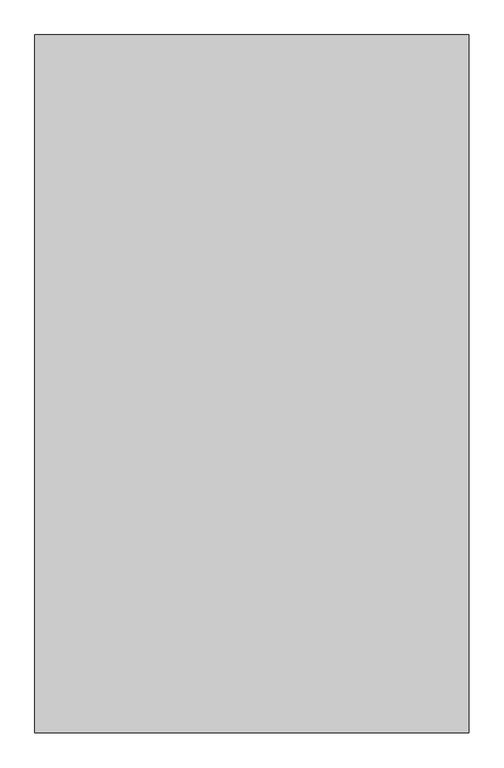
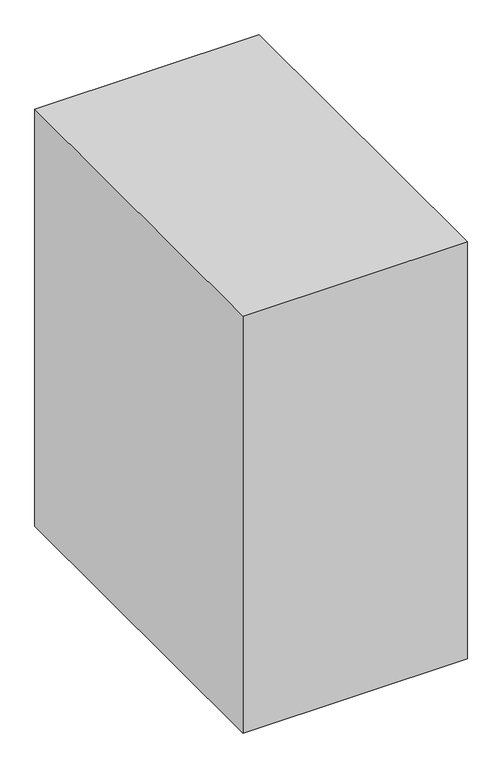
"""IFC4 building model written with IfcOpenShell, lengths in millimetres: proxy geometry, Space Planning Box_hec : Space Planning Box_hec."""

import ifcopenshell
import ifcopenshell.guid

model = None  # the IFC model being written
_history = None  # IfcOwnerHistory: only IFC2X3 demands one
_inside = {}  # id of a spatial element -> (the spatial element, [elements in it])
_under = {}  # id of a project, library or spatial element -> (it, [spatial elements below it])
_declared = {}  # id of a project -> (the project, [libraries it declares])
_typed = {}  # id of a type object -> (the type object, [elements of that type])
_made_of = {}  # id of a material, layer set ... -> (it, [elements and type objects made of it])


def new_model(schema):
    """Start an empty IFC model of exactly this schema.

    Asked for "IFC4X3", IfcOpenShell would pick the latest addendum, in which some entities
    have other attributes; the version numbers below select the first issue.
    IFC2X3 requires an IfcOwnerHistory on every rooted entity: one is made here for all.
    """
    global model, _history
    if schema == "IFC4X3":
        model = ifcopenshell.file(schema_version=(4, 3, 0, 0))
    else:
        model = ifcopenshell.file(schema=schema)
    _inside.clear()
    _under.clear()
    _declared.clear()
    _typed.clear()
    _made_of.clear()
    _history = None
    if model.schema == "IFC2X3":
        org = make("IfcOrganization", Name="unknown")
        user = make(
            "IfcPersonAndOrganization",
            ThePerson=make("IfcPerson", FamilyName="unknown"),
            TheOrganization=org,
        )
        app = make(
            "IfcApplication",
            ApplicationDeveloper=org,
            Version="unknown",
            ApplicationFullName="unknown",
            ApplicationIdentifier="unknown",
        )
        _history = make(
            "IfcOwnerHistory",
            OwningUser=user,
            OwningApplication=app,
            ChangeAction="ADDED",
            CreationDate=0,
        )
    return model


def make(cls, **values):
    """One entity of the class cls with the attributes given. An attribute that is None is left unset."""
    return model.create_entity(
        cls, **{name: value for name, value in values.items() if value is not None}
    )


def rooted(cls, **values):
    """An entity with a GlobalId (a new one), such as an element, a storey or a relation."""
    return make(cls, GlobalId=ifcopenshell.guid.new(), OwnerHistory=_history, **values)


def si_unit(unit_type, name, prefix=None):
    """IfcSIUnit, for example si_unit("LENGTHUNIT", "METRE", prefix="MILLI")."""
    return make("IfcSIUnit", UnitType=unit_type, Prefix=prefix, Name=name)


def assignment(units):
    """IfcUnitAssignment: the units of a project."""
    return None if units is None else make("IfcUnitAssignment", Units=units)


def point(xyz):
    """IfcCartesianPoint."""
    return None if xyz is None else make("IfcCartesianPoint", Coordinates=xyz)


def direction(xyz):
    """IfcDirection."""
    return None if xyz is None else make("IfcDirection", DirectionRatios=xyz)


def frame(location, z_axis=None, x_axis=None):
    """IfcAxis2Placement3D, a coordinate frame: its origin and axes. An axis left out is left unset."""
    return make(
        "IfcAxis2Placement3D",
        Location=point(location),
        Axis=direction(z_axis),
        RefDirection=direction(x_axis),
    )


def origin():
    """The frame at (0, 0, 0) with its axes left unset."""
    return frame((0.0, 0.0, 0.0))


def origin_with_axes():
    """The frame at (0, 0, 0) with the z axis (0, 0, 1) and the x axis (1, 0, 0) written out."""
    return frame((0.0, 0.0, 0.0), z_axis=(0.0, 0.0, 1.0), x_axis=(1.0, 0.0, 0.0))


def place(relative_to, where):
    """IfcLocalPlacement: puts the frame where relative to a parent placement (None: the world)."""
    return make(
        "IfcLocalPlacement", PlacementRelTo=relative_to, RelativePlacement=where
    )


def context(
    kind, dimensions, precision=None, world=None, true_north=None, identifier=None
):
    """IfcGeometricRepresentationContext, for example the 3D "Model" context."""
    return make(
        "IfcGeometricRepresentationContext",
        ContextIdentifier=identifier,
        ContextType=kind,
        CoordinateSpaceDimension=dimensions,
        Precision=precision,
        WorldCoordinateSystem=world,
        TrueNorth=true_north,
    )


def project(units=None, contexts=None):
    """IfcProject with its units and contexts."""
    return rooted(
        "IfcProject",
        Name="project",
        RepresentationContexts=contexts,
        UnitsInContext=assignment(units),
    )


def spatial(cls, under=None, at=None, **own):
    """A site, building, storey or space (cls), placed at a placement, below another one or the project."""
    s = rooted(cls, ObjectPlacement=at, **own)
    if under is not None:
        _under.setdefault(under.id(), (under, []))[1].append(s)
    return s


def polyline(points):
    """IfcPolyline through the points."""
    return make("IfcPolyline", Points=[point(p) for p in points])


def outline(outer, holes=None, kind="AREA"):
    """IfcArbitraryClosedProfileDef: a profile drawn as a closed curve; with holes, ...WithVoids."""
    if holes is None:
        return make("IfcArbitraryClosedProfileDef", ProfileType=kind, OuterCurve=outer)
    return make(
        "IfcArbitraryProfileDefWithVoids",
        ProfileType=kind,
        OuterCurve=outer,
        InnerCurves=holes,
    )


def extrude(swept, where, along, depth):
    """IfcExtrudedAreaSolid: the profile swept, set in the frame where, extruded along a direction by depth."""
    return make(
        "IfcExtrudedAreaSolid",
        SweptArea=swept,
        Position=where,
        ExtrudedDirection=direction(along),
        Depth=depth,
    )


def shape(context_of_items, identifier, shape_type, items):
    """IfcShapeRepresentation: the items that make up one representation, for example the "Body"."""
    return make(
        "IfcShapeRepresentation",
        ContextOfItems=context_of_items,
        RepresentationIdentifier=identifier,
        RepresentationType=shape_type,
        Items=items,
    )


def source(mapping_origin, context_of_items, identifier, shape_type, items):
    """IfcRepresentationMap: a shape defined once, which mapped items show again and again."""
    return make(
        "IfcRepresentationMap",
        MappingOrigin=mapping_origin,
        MappedRepresentation=shape(context_of_items, identifier, shape_type, items),
    )


def transform(
    local_origin,
    x_axis=None,
    y_axis=None,
    z_axis=None,
    scale=None,
    scale2=None,
    scale3=None,
    uniform=True,
):
    """IfcCartesianTransformationOperator3D, or its non-uniform kind. x_axis, y_axis, z_axis: its Axis1, 2, 3."""
    if uniform:
        return make(
            "IfcCartesianTransformationOperator3D",
            Axis1=direction(x_axis),
            Axis2=direction(y_axis),
            LocalOrigin=point(local_origin),
            Scale=scale,
            Axis3=direction(z_axis),
        )
    return make(
        "IfcCartesianTransformationOperator3DnonUniform",
        Axis1=direction(x_axis),
        Axis2=direction(y_axis),
        LocalOrigin=point(local_origin),
        Scale=scale,
        Axis3=direction(z_axis),
        Scale2=scale2,
        Scale3=scale3,
    )


def mapped(mapping_source, mapping_target):
    """IfcMappedItem: shows the shape of a source again, moved by a transform."""
    return make(
        "IfcMappedItem", MappingSource=mapping_source, MappingTarget=mapping_target
    )


def made_of(thing, what):
    """Note that an element or type object is made of a material, layer set ...; save() writes the relation."""
    if what is not None:
        _made_of.setdefault(what.id(), (what, []))[1].append(thing)
    return thing


def element(
    cls,
    number,
    at=None,
    inside=None,
    cuts=None,
    type_object=None,
    material=None,
    context=None,
    identifier="Body",
    shape_type=None,
    held_by="IfcProductDefinitionShape",
    body=None,
    shapes=None,
    **own,
):
    """One element of the class cls, such as IfcWall. Its Tag is "e" and its number.

    at: its placement. inside: the storey or other place that contains it. cuts: it is an
    opening in that element (IfcRelVoidsElement). A single representation is given by context,
    identifier, shape_type and body (its items); several are given by shapes. held_by: the class
    of the entity that holds the representations. save() writes the other relations.
    """
    e = rooted(cls, Tag="e%d" % number, ObjectPlacement=at, **own)
    if body is not None:
        shapes = [shape(context, identifier, shape_type, body)]
    if shapes is not None:
        e.Representation = make(held_by, Representations=shapes)
    if inside is not None:
        _inside.setdefault(inside.id(), (inside, []))[1].append(e)
    if cuts is not None:
        rooted(
            "IfcRelVoidsElement", RelatingBuildingElement=cuts, RelatedOpeningElement=e
        )
    if type_object is not None:
        _typed.setdefault(type_object.id(), (type_object, []))[1].append(e)
    return made_of(e, material)


def aggregate(whole, parts):
    """IfcRelAggregates: a whole, such as a stair, and the parts it consists of."""
    return rooted("IfcRelAggregates", RelatingObject=whole, RelatedObjects=parts)


def save(model, path):
    """Write the relations noted so far, then the file.

    IfcRelAggregates (storeys below a building ...), IfcRelContainedInSpatialStructure (elements
    in a storey), IfcRelDefinesByType, IfcRelAssociatesMaterial and IfcRelDeclares: one each for
    every whole, place, type object, material and project.
    """
    for whole, parts in _under.values():
        aggregate(whole, parts)
    for where, things in _inside.values():
        rooted(
            "IfcRelContainedInSpatialStructure",
            RelatedElements=things,
            RelatingStructure=where,
        )
    for kind, things in _typed.values():
        rooted("IfcRelDefinesByType", RelatedObjects=things, RelatingType=kind)
    for what, things in _made_of.values():
        rooted("IfcRelAssociatesMaterial", RelatedObjects=things, RelatingMaterial=what)
    for by, libraries in _declared.values():
        rooted("IfcRelDeclares", RelatingContext=by, RelatedDefinitions=libraries)
    model.write(path)


def generic_models_ac48a1a3(model_context):
    return source(origin(), model_context, "Body", "SweptSolid", [
        extrude(outline(polyline([(1400.0, 2250.0), (1400.0, -2250.0), (-1400.0, -2250.0), (-1400.0, 2250.0), (1400.0, 2250.0)])), origin_with_axes(), (0.0, 0.0, 1.0), 5500.0),
    ])


if __name__ == "__main__":
    model = new_model("IFC4")
    model_context = context("Model", 3, world=origin())
    ifc_project = project(units=[si_unit("LENGTHUNIT", "METRE", prefix="MILLI")], contexts=[model_context])
    site = spatial("IfcSite", under=ifc_project)
    building = spatial("IfcBuilding", under=site)
    placement = place(None, origin())
    generic_models_shape = generic_models_ac48a1a3(model_context)
    element("IfcBuildingElementProxy", 1, Name="Space Planning Box_hec : Space Planning Box_hec", ObjectType="Space Planning Box_hec : Space Planning Box_hec", at=placement, inside=building, context=model_context, shape_type="MappedRepresentation", body=[
        mapped(generic_models_shape, transform((0.0, 0.0, 0.0), x_axis=(1.0, 0.0, 0.0), y_axis=(0.0, 1.0, 0.0), z_axis=(0.0, 0.0, 1.0))),
    ])
    save(model, "model.ifc")

# Revit data of these elements
# Type "Space Planning Box_hec : Space Planning Box_hec"
#   Type Comments = "..."
#   Room Name [instance default] = "?"
#   Interior Finish [instance default] = ""
#   Exterior Finish [instance default] = ""
#   Department [instance default] = ""
#   Assembly Code = "..."
#   ceiling height [instance default] = 0
#   Width [instance default] = 1524 mm
#   Program Area [instance default] = 0.00 m²
#   Length [instance default] = 1524 mm
#   Height [instance default] = 1524 mm
#   Area [instance default] = 2.32258 m²
#   Fill Color [instance default] = Cyan
#   Default Elevation = 0
# Element 1 (IfcBuildingElementProxy, "Space Planning Box_hec : Space Planning Box_hec")
#   Room Name = "Toilet"
#   Exterior Finish = "N/A..N/A,,EW2..N/A..N/A"
#   Department = "AR"
#   Width = 2800 mm
#   Program Area = 12.60 m²
#   Length = 4500 mm
#   Height = 5500 mm
#   Area = 12.60 m²
#   Materials on its faces: "Cyan"
# Materials
#   "Cyan": class "Generic", colour RGB 0 255 255, transparency 0.2, Cost = 0
